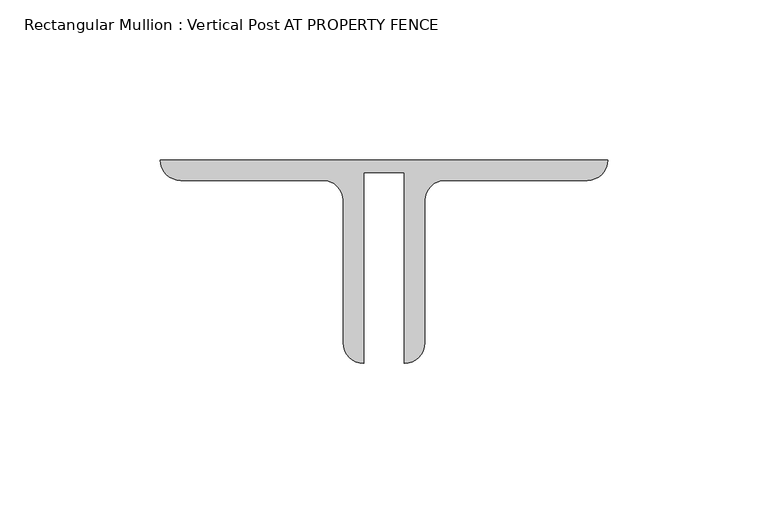
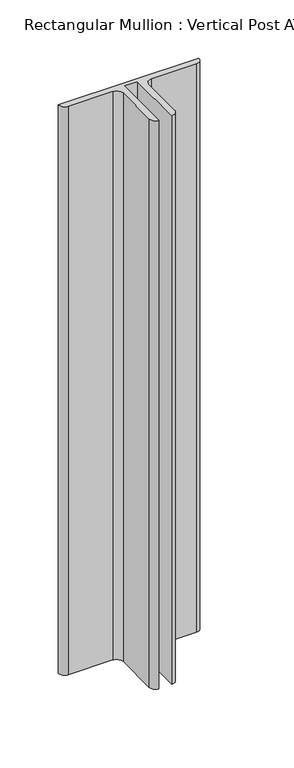
"""IFC4 building model written with IfcOpenShell, lengths in millimetres: member geometry, Rectangular Mullion : Vertical Post AT PROPERTY FENCE."""

from ifc_helpers import new_model, si_unit, point, frame, frame_2d, origin, place, context, project, spatial, polyline, circle_curve, trimmed, segment, composite_curve, outline, extrude, source, transform, mapped, element, save


def rectangular_mullion_vertical_post_at_property_fence_ea6aaa4f(model_context):
    return source(origin(), model_context, "Body", "SweptSolid", [
        extrude(outline(composite_curve([segment(polyline([(-6.35, -22.9145205), (-6.35, -82.55)]), True, "CONTINUOUS"), segment(trimmed(circle_curve(frame_2d((-6.35, -76.2)), 6.35), [point((-6.35, -82.55))], [point((-12.7, -76.2))], False, "CARTESIAN"), True, "CONTINUOUS"), segment(polyline([(-12.7, -76.2), (-12.7, -31.75)]), True, "CONTINUOUS"), segment(trimmed(circle_curve(frame_2d((-19.05, -31.75)), 6.35), [point((-12.7, -31.75))], [point((-19.05, -25.4))], True, "CARTESIAN"), True, "CONTINUOUS"), segment(polyline([(-19.05, -25.4), (-63.5, -25.4)]), True, "CONTINUOUS"), segment(trimmed(circle_curve(frame_2d((-63.5, -19.05)), 6.35), [point((-63.5, -25.4))], [point((-69.85, -19.05))], False, "CARTESIAN"), True, "CONTINUOUS"), segment(polyline([(-69.85, -19.05), (69.85, -19.05)]), True, "CONTINUOUS"), segment(trimmed(circle_curve(frame_2d((63.5, -19.05)), 6.35), [point((69.85, -19.05))], [point((63.5, -25.4))], False, "CARTESIAN"), True, "CONTINUOUS"), segment(polyline([(63.5, -25.4), (19.05, -25.4)]), True, "CONTINUOUS"), segment(trimmed(circle_curve(frame_2d((19.05, -31.75)), 6.35), [point((19.05, -25.4))], [point((12.7, -31.75))], True, "CARTESIAN"), True, "CONTINUOUS"), segment(polyline([(12.7, -31.75), (12.7, -76.2)]), True, "CONTINUOUS"), segment(trimmed(circle_curve(frame_2d((6.35, -76.2)), 6.35), [point((12.7, -76.2))], [point((6.35, -82.55))], False, "CARTESIAN"), True, "CONTINUOUS"), segment(polyline([(6.35, -82.55), (6.35, -22.9145205), (-6.35, -22.9145205)]), True, "CONTINUOUS")], self_intersect=False)), frame((0.0, 0.0, -596.9), z_axis=(0.0, 0.0, 1.0), x_axis=(1.0, 0.0, 0.0)), (0.0, 0.0, 1.0), 596.9),
    ])


if __name__ == "__main__":
    model = new_model("IFC4")
    model_context = context("Model", 3, world=origin())
    ifc_project = project(units=[si_unit("LENGTHUNIT", "METRE", prefix="MILLI")], contexts=[model_context])
    site = spatial("IfcSite", under=ifc_project)
    building = spatial("IfcBuilding", under=site)
    placement = place(None, origin())
    rectangular_mullion_vertical_post_at_property_fence_shape = rectangular_mullion_vertical_post_at_property_fence_ea6aaa4f(model_context)
    element("IfcMember", 1, ObjectType="Rectangular Mullion : Vertical Post AT PROPERTY FENCE", at=placement, inside=building, context=model_context, shape_type="MappedRepresentation", body=[
        mapped(rectangular_mullion_vertical_post_at_property_fence_shape, transform((0.0, 0.0, 0.0), x_axis=(1.0, 0.0, 0.0), y_axis=(0.0, 1.0, 0.0), z_axis=(0.0, 0.0, 1.0))),
    ])
    save(model, "model.ifc")

# Revit data of these elements
# Type "Rectangular Mullion : Vertical Post AT PROPERTY FENCE"
#   built-in parameter 1007351 = -0.0625 (stored number, unit not read)
#   built-in parameter 1007322 = 0.0126789 (stored number, unit not read)
#   built-in parameter 1007321 = 0.229167 (stored number, unit not read)
#   built-in parameter 1007320 = 0.229167 (stored number, unit not read)
# Element 1 (IfcMember, "Rectangular Mullion : Vertical Post AT PROPERTY FENCE")
#   Materials on its faces: "MAIN FENCE POST: (2) BACK/BACK GALVANIZED ANGLES (2) L2 1/2 X 2 1/2 X 1/4\") ANCHORED TO 8\"W X 42\" DEEP CONCRETE FOOTING(1)"
# Materials
#   "MAIN FENCE POST: (2) BACK/BACK GALVANIZED ANGLES (2) L2 1/2 X 2 1/2 X 1/4\") ANCHORED TO 8\"W X 42\" DEEP CONCRETE FOOTING(1)": class "Unassigned", colour RGB 211 211 211, transparency 0, Cost = 0
